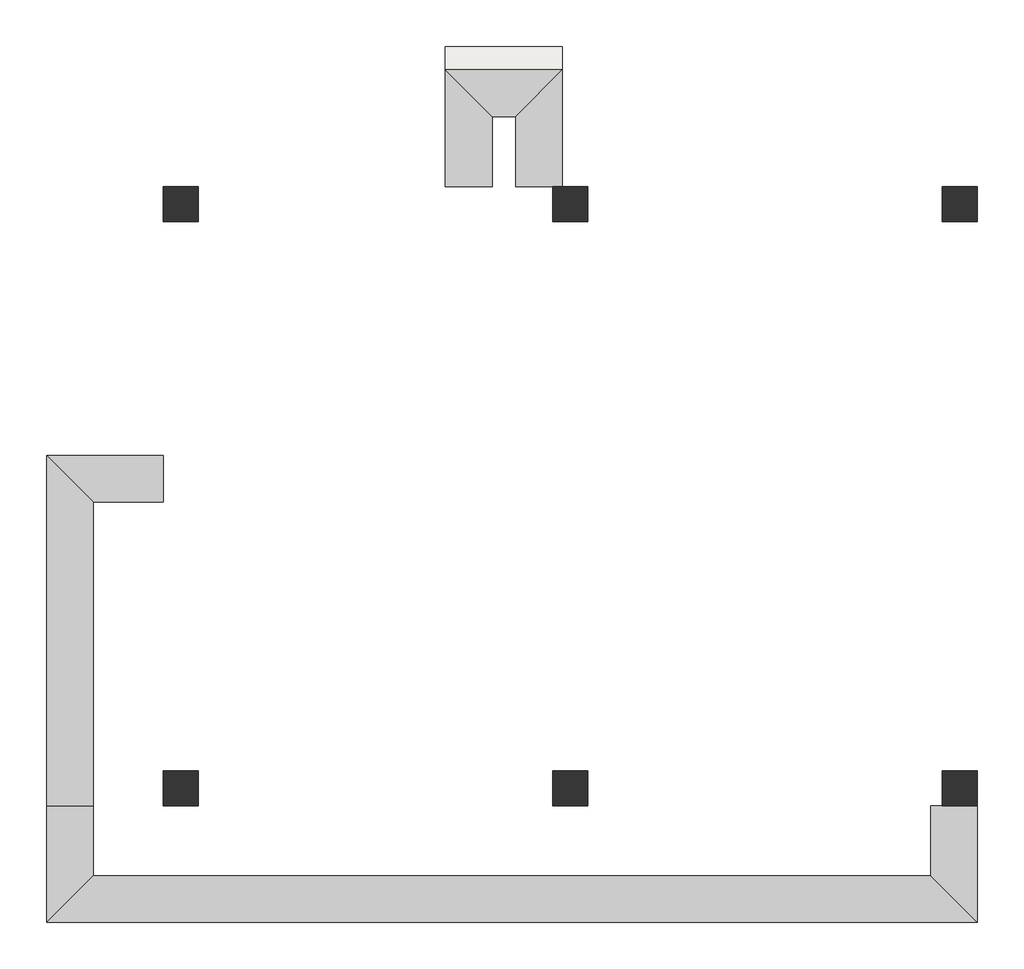
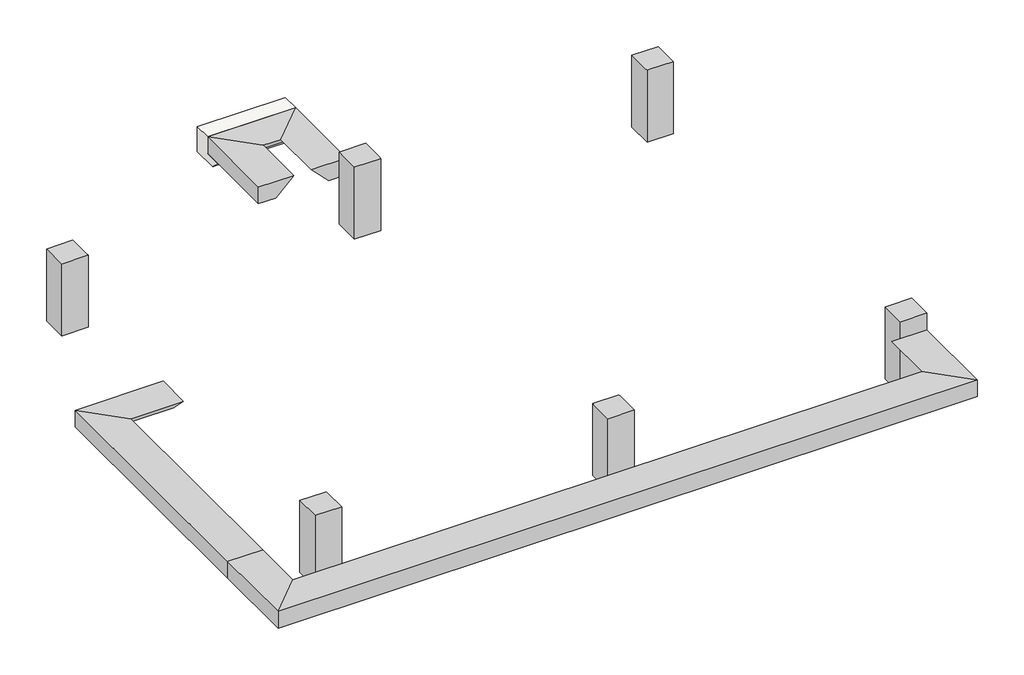
# One storey: 6 columns, 2 proxies, 1 slab.
"""IFC4 building model written with IfcOpenShell, lengths in millimetres."""

import ifcopenshell
import ifcopenshell.guid

model = None  # the IFC model being written
_history = None  # IfcOwnerHistory: only IFC2X3 demands one
_inside = {}  # id of a spatial element -> (the spatial element, [elements in it])
_under = {}  # id of a project, library or spatial element -> (it, [spatial elements below it])
_declared = {}  # id of a project -> (the project, [libraries it declares])
_typed = {}  # id of a type object -> (the type object, [elements of that type])
_made_of = {}  # id of a material, layer set ... -> (it, [elements and type objects made of it])


def new_model(schema):
    """Start an empty IFC model of exactly this schema.

    Asked for "IFC4X3", IfcOpenShell would pick the latest addendum, in which some entities
    have other attributes; the version numbers below select the first issue.
    IFC2X3 requires an IfcOwnerHistory on every rooted entity: one is made here for all.
    """
    global model, _history
    if schema == "IFC4X3":
        model = ifcopenshell.file(schema_version=(4, 3, 0, 0))
    else:
        model = ifcopenshell.file(schema=schema)
    _inside.clear()
    _under.clear()
    _declared.clear()
    _typed.clear()
    _made_of.clear()
    _history = None
    if model.schema == "IFC2X3":
        org = make("IfcOrganization", Name="unknown")
        user = make(
            "IfcPersonAndOrganization",
            ThePerson=make("IfcPerson", FamilyName="unknown"),
            TheOrganization=org,
        )
        app = make(
            "IfcApplication",
            ApplicationDeveloper=org,
            Version="unknown",
            ApplicationFullName="unknown",
            ApplicationIdentifier="unknown",
        )
        _history = make(
            "IfcOwnerHistory",
            OwningUser=user,
            OwningApplication=app,
            ChangeAction="ADDED",
            CreationDate=0,
        )
    return model


def make(cls, **values):
    """One entity of the class cls with the attributes given. An attribute that is None is left unset."""
    return model.create_entity(
        cls, **{name: value for name, value in values.items() if value is not None}
    )


def rooted(cls, **values):
    """An entity with a GlobalId (a new one), such as an element, a storey or a relation."""
    return make(cls, GlobalId=ifcopenshell.guid.new(), OwnerHistory=_history, **values)


def si_unit(unit_type, name, prefix=None):
    """IfcSIUnit, for example si_unit("LENGTHUNIT", "METRE", prefix="MILLI")."""
    return make("IfcSIUnit", UnitType=unit_type, Prefix=prefix, Name=name)


def assignment(units):
    """IfcUnitAssignment: the units of a project."""
    return None if units is None else make("IfcUnitAssignment", Units=units)


def point(xyz):
    """IfcCartesianPoint."""
    return None if xyz is None else make("IfcCartesianPoint", Coordinates=xyz)


def direction(xyz):
    """IfcDirection."""
    return None if xyz is None else make("IfcDirection", DirectionRatios=xyz)


def frame(location, z_axis=None, x_axis=None):
    """IfcAxis2Placement3D, a coordinate frame: its origin and axes. An axis left out is left unset."""
    return make(
        "IfcAxis2Placement3D",
        Location=point(location),
        Axis=direction(z_axis),
        RefDirection=direction(x_axis),
    )


def origin():
    """The frame at (0, 0, 0) with its axes left unset."""
    return frame((0.0, 0.0, 0.0))


def place(relative_to, where):
    """IfcLocalPlacement: puts the frame where relative to a parent placement (None: the world)."""
    return make(
        "IfcLocalPlacement", PlacementRelTo=relative_to, RelativePlacement=where
    )


def context(
    kind, dimensions, precision=None, world=None, true_north=None, identifier=None
):
    """IfcGeometricRepresentationContext, for example the 3D "Model" context."""
    return make(
        "IfcGeometricRepresentationContext",
        ContextIdentifier=identifier,
        ContextType=kind,
        CoordinateSpaceDimension=dimensions,
        Precision=precision,
        WorldCoordinateSystem=world,
        TrueNorth=true_north,
    )


def project(units=None, contexts=None):
    """IfcProject with its units and contexts."""
    return rooted(
        "IfcProject",
        Name="project",
        RepresentationContexts=contexts,
        UnitsInContext=assignment(units),
    )


def spatial(cls, under=None, at=None, **own):
    """A site, building, storey or space (cls), placed at a placement, below another one or the project."""
    s = rooted(cls, ObjectPlacement=at, **own)
    if under is not None:
        _under.setdefault(under.id(), (under, []))[1].append(s)
    return s


def polyline(points):
    """IfcPolyline through the points."""
    return make("IfcPolyline", Points=[point(p) for p in points])


def outline(outer, holes=None, kind="AREA"):
    """IfcArbitraryClosedProfileDef: a profile drawn as a closed curve; with holes, ...WithVoids."""
    if holes is None:
        return make("IfcArbitraryClosedProfileDef", ProfileType=kind, OuterCurve=outer)
    return make(
        "IfcArbitraryProfileDefWithVoids",
        ProfileType=kind,
        OuterCurve=outer,
        InnerCurves=holes,
    )


def extrude(swept, where, along, depth):
    """IfcExtrudedAreaSolid: the profile swept, set in the frame where, extruded along a direction by depth."""
    return make(
        "IfcExtrudedAreaSolid",
        SweptArea=swept,
        Position=where,
        ExtrudedDirection=direction(along),
        Depth=depth,
    )


def faces_of(points, faces, orient=None, outer=None):
    """IfcFace entities. A face is a list of loops; a loop is a list of indices into points, from 0.

    orient and outer hold one flag for each loop. By default every Orientation is true, the
    first loop of a face is its IfcFaceOuterBound and the others are IfcFaceBound.
    """
    made = []
    for i, loops in enumerate(faces):
        bounds = []
        for j, loop in enumerate(loops):
            is_outer = j == 0 if outer is None else outer[i][j]
            bounds.append(
                make(
                    "IfcFaceOuterBound" if is_outer else "IfcFaceBound",
                    Bound=make("IfcPolyLoop", Polygon=[points[k] for k in loop]),
                    Orientation=True if orient is None else orient[i][j],
                )
            )
        made.append(make("IfcFace", Bounds=bounds))
    return made


def faceted_brep(points, faces, orient=None, outer=None, voids=None):
    """IfcFacetedBrep: a solid bounded by flat faces; with voids (closed shells), ...WithVoids."""
    shared = [point(p) for p in points]
    hull = make("IfcClosedShell", CfsFaces=faces_of(shared, faces, orient, outer))
    if voids is None:
        return make("IfcFacetedBrep", Outer=hull)
    return make(
        "IfcFacetedBrepWithVoids",
        Outer=hull,
        Voids=[
            make(cls, CfsFaces=faces_of(shared, fs, o, b)) for cls, fs, o, b in voids
        ],
    )


def shape(context_of_items, identifier, shape_type, items):
    """IfcShapeRepresentation: the items that make up one representation, for example the "Body"."""
    return make(
        "IfcShapeRepresentation",
        ContextOfItems=context_of_items,
        RepresentationIdentifier=identifier,
        RepresentationType=shape_type,
        Items=items,
    )


def made_of(thing, what):
    """Note that an element or type object is made of a material, layer set ...; save() writes the relation."""
    if what is not None:
        _made_of.setdefault(what.id(), (what, []))[1].append(thing)
    return thing


def element(
    cls,
    number,
    at=None,
    inside=None,
    cuts=None,
    type_object=None,
    material=None,
    context=None,
    identifier="Body",
    shape_type=None,
    held_by="IfcProductDefinitionShape",
    body=None,
    shapes=None,
    **own,
):
    """One element of the class cls, such as IfcWall. Its Tag is "e" and its number.

    at: its placement. inside: the storey or other place that contains it. cuts: it is an
    opening in that element (IfcRelVoidsElement). A single representation is given by context,
    identifier, shape_type and body (its items); several are given by shapes. held_by: the class
    of the entity that holds the representations. save() writes the other relations.
    """
    e = rooted(cls, Tag="e%d" % number, ObjectPlacement=at, **own)
    if body is not None:
        shapes = [shape(context, identifier, shape_type, body)]
    if shapes is not None:
        e.Representation = make(held_by, Representations=shapes)
    if inside is not None:
        _inside.setdefault(inside.id(), (inside, []))[1].append(e)
    if cuts is not None:
        rooted(
            "IfcRelVoidsElement", RelatingBuildingElement=cuts, RelatedOpeningElement=e
        )
    if type_object is not None:
        _typed.setdefault(type_object.id(), (type_object, []))[1].append(e)
    return made_of(e, material)


def aggregate(whole, parts):
    """IfcRelAggregates: a whole, such as a stair, and the parts it consists of."""
    return rooted("IfcRelAggregates", RelatingObject=whole, RelatedObjects=parts)


def save(model, path):
    """Write the relations noted so far, then the file.

    IfcRelAggregates (storeys below a building ...), IfcRelContainedInSpatialStructure (elements
    in a storey), IfcRelDefinesByType, IfcRelAssociatesMaterial and IfcRelDeclares: one each for
    every whole, place, type object, material and project.
    """
    for whole, parts in _under.values():
        aggregate(whole, parts)
    for where, things in _inside.values():
        rooted(
            "IfcRelContainedInSpatialStructure",
            RelatedElements=things,
            RelatingStructure=where,
        )
    for kind, things in _typed.values():
        rooted("IfcRelDefinesByType", RelatedObjects=things, RelatingType=kind)
    for what, things in _made_of.values():
        rooted("IfcRelAssociatesMaterial", RelatedObjects=things, RelatingMaterial=what)
    for by, libraries in _declared.values():
        rooted("IfcRelDeclares", RelatingContext=by, RelatedDefinitions=libraries)
    model.write(path)


model = new_model("IFC4")

# Units and contexts
model_context = context("Model", 3, world=origin())
ifc_project = project(units=[si_unit("LENGTHUNIT", "METRE", prefix="MILLI")], contexts=[model_context])

# Site, building, storey
site = spatial("IfcSite", under=ifc_project)
building = spatial("IfcBuilding", under=site)
storey = spatial("IfcBuildingStorey", under=building, Name="T.O.C_-1,300", Elevation=-1300.0)

# Proxies
placement = place(None, origin())
element("IfcBuildingElementProxy", 1, Name="Slab Edge", ObjectType="Slab Edge", at=placement, inside=storey, context=model_context, shape_type="Brep", body=[
    faceted_brep([(10225.0, 13274.5208589, -600.0), (9925.0, 13274.5208589, -600.0), (9625.0, 13274.5208589, -300.0), (10225.0, 13274.5208589, -300.0), (10225.0, 11774.5208589, -300.0), (10225.0, 11774.5208589, -600.0), (9625.0, 12374.5208589, -300.0), (9925.0, 12074.5208589, -600.0), (-1725.0, 11774.5208589, -300.0), (-1725.0, 11774.5208589, -600.0), (-1125.0, 12374.5208589, -300.0), (-1425.0, 12074.5208589, -600.0), (-1725.0, 17774.5208589, -300.0), (-1725.0, 17774.5208589, -600.0), (-1725.0, 13274.5208589, -600.0), (-1725.0, 13274.5208589, -300.0), (-1125.0, 17174.5208589, -300.0), (-1125.0, 13274.5208589, -300.0), (-1425.0, 17474.5208589, -600.0), (-1425.0, 13274.5208589, -600.0), (-225.0, 17774.5208589, -600.0), (-225.0, 17774.5208589, -300.0), (-225.0, 17174.5208589, -300.0), (-225.0, 17474.5208589, -600.0)], [[[0, 1, 2, 3]], [[4, 5, 0, 3]], [[6, 4, 3, 2]], [[7, 6, 2, 1]], [[5, 7, 1, 0]], [[8, 9, 5, 4]], [[10, 8, 4, 6]], [[11, 10, 6, 7]], [[9, 11, 7, 5]], [[12, 13, 14, 15]], [[16, 12, 15, 17]], [[18, 16, 17, 19]], [[13, 18, 19, 14]], [[15, 14, 9, 8]], [[17, 15, 8, 10]], [[19, 17, 10, 11]], [[14, 19, 11, 9]], [[20, 21, 22, 23]], [[21, 20, 13, 12]], [[22, 21, 12, 16]], [[23, 22, 16, 18]], [[20, 23, 18, 13]]]),
])
element("IfcBuildingElementProxy", 2, Name="Slab Edge", ObjectType="Slab Edge", at=placement, inside=storey, context=model_context, shape_type="Brep", body=[
    faceted_brep([(4895.0, 21224.5208589, -450.0), (4895.0, 21224.5208589, -150.0), (4295.0, 21224.5208589, -150.0), (4595.0, 21224.5208589, -450.0), (4895.0, 22724.5208589, -450.0), (4895.0, 22724.5208589, -150.0), (4295.0, 22124.5208589, -150.0), (4595.0, 22424.5208589, -450.0), (3395.0, 22724.5208589, -450.0), (3395.0, 22724.5208589, -150.0), (3995.0, 22124.5208589, -150.0), (3695.0, 22424.5208589, -450.0), (3395.0, 21224.5208589, -450.0), (3695.0, 21224.5208589, -450.0), (3995.0, 21224.5208589, -150.0), (3395.0, 21224.5208589, -150.0)], [[[0, 1, 2, 3]], [[1, 0, 4, 5]], [[2, 1, 5, 6]], [[3, 2, 6, 7]], [[0, 3, 7, 4]], [[5, 4, 8, 9]], [[6, 5, 9, 10]], [[7, 6, 10, 11]], [[4, 7, 11, 8]], [[12, 13, 14, 15]], [[9, 8, 12, 15]], [[10, 9, 15, 14]], [[11, 10, 14, 13]], [[8, 11, 13, 12]]]),
])

# Columns
element("IfcColumn", 3, ObjectType="Concrete-Rectangular-Column : CL111_450x450", at=placement, inside=storey, context=model_context, shape_type="Brep", body=[
    faceted_brep([(225.0, 13724.5208589, -1300.0), (225.0, 13274.5208589, -1300.0), (-225.0, 13274.5208589, -1300.0), (-225.0, 13724.5208589, -1300.0), (225.0, 13724.5208589, 0.0), (225.0, 13674.5208589, 0.0), (225.0, 13274.5208589, 0.0), (225.0, 13274.5208589, -600.0), (-225.0, 13274.5208589, 0.0), (-225.0, 13724.5208589, 0.0), (-225.0, 13724.5208589, -600.0), (175.0, 13724.5208589, 0.0)], [[[0, 1, 2, 3]], [[4, 5, 6, 7, 1, 0]], [[6, 8, 2, 1, 7]], [[8, 9, 10, 3, 2]], [[9, 11, 4, 0, 3, 10]], [[4, 11, 9, 8, 6, 5]]]),
])
element("IfcColumn", 4, ObjectType="Concrete-Rectangular-Column : CL111_450x450", at=placement, inside=storey, context=model_context, shape_type="Brep", body=[
    faceted_brep([(5225.0, 13724.5208589, -1300.0), (5225.0, 13274.5208589, -1300.0), (4775.0, 13274.5208589, -1300.0), (4775.0, 13724.5208589, -1300.0), (5225.0, 13724.5208589, 0.0), (5225.0, 13674.5208589, 0.0), (5225.0, 13274.5208589, 0.0), (5225.0, 13274.5208589, -600.0), (4775.0, 13274.5208589, 0.0), (4775.0, 13274.5208589, -600.0), (4775.0, 13674.5208589, 0.0), (4775.0, 13724.5208589, 0.0)], [[[0, 1, 2, 3]], [[4, 5, 6, 7, 1, 0]], [[6, 8, 9, 2, 1, 7]], [[8, 10, 11, 3, 2, 9]], [[11, 4, 0, 3]], [[4, 11, 10, 8, 6, 5]]]),
])
element("IfcColumn", 5, ObjectType="Concrete-Rectangular-Column : CL111_450x450", at=placement, inside=storey, context=model_context, shape_type="Brep", body=[
    faceted_brep([(10225.0, 13724.5208589, -1300.0), (10225.0, 13274.5208589, -1300.0), (9775.0, 13274.5208589, -1300.0), (9775.0, 13724.5208589, -1300.0), (10225.0, 13724.5208589, 0.0), (10225.0, 13274.5208589, 0.0), (10225.0, 13724.5208589, -600.0), (9775.0, 13274.5208589, 0.0), (9775.0, 13274.5208589, -600.0), (9775.0, 13674.5208589, 0.0), (9775.0, 13724.5208589, 0.0), (9825.0, 13724.5208589, 0.0)], [[[0, 1, 2, 3]], [[4, 5, 1, 0, 6]], [[5, 7, 8, 2, 1]], [[7, 9, 10, 3, 2, 8]], [[10, 11, 4, 6, 0, 3]], [[4, 11, 10, 9, 7, 5]]]),
])
element("IfcColumn", 6, ObjectType="Concrete-Rectangular-Column : CL111_450x450", at=placement, inside=storey, context=model_context, shape_type="Brep", body=[
    faceted_brep([(10225.0, 21224.5208589, -1300.0), (10225.0, 20774.5208589, -1300.0), (9775.0, 20774.5208589, -1300.0), (9775.0, 21224.5208589, -1300.0), (10225.0, 21224.5208589, 0.0), (10225.0, 20774.5208589, 0.0), (10225.0, 20774.5208589, -600.0), (9825.0, 20774.5208589, 0.0), (9775.0, 20774.5208589, 0.0), (9775.0, 20824.5208589, 0.0), (9775.0, 21224.5208589, 0.0), (9775.0, 21224.5208589, -600.0)], [[[0, 1, 2, 3]], [[4, 5, 6, 1, 0]], [[5, 7, 8, 2, 1, 6]], [[8, 9, 10, 11, 3, 2]], [[10, 4, 0, 3, 11]], [[4, 10, 9, 8, 7, 5]]]),
])
element("IfcColumn", 7, ObjectType="Concrete-Rectangular-Column : CL111_450x450", at=placement, inside=storey, context=model_context, shape_type="Brep", body=[
    faceted_brep([(5225.0, 21224.5208589, -1300.0), (5225.0, 20774.5208589, -1300.0), (4775.0, 20774.5208589, -1300.0), (4775.0, 21224.5208589, -1300.0), (5225.0, 21224.5208589, 0.0), (5225.0, 20824.5208589, 0.0), (5225.0, 20774.5208589, 0.0), (5225.0, 21224.5208589, -600.0), (4775.0, 20774.5208589, 0.0), (4775.0, 21224.5208589, 0.0)], [[[0, 1, 2, 3]], [[4, 5, 6, 1, 0, 7]], [[6, 8, 2, 1]], [[8, 9, 3, 2]], [[9, 4, 7, 0, 3]], [[4, 9, 8, 6, 5]]]),
])
element("IfcColumn", 8, ObjectType="Concrete-Rectangular-Column : CL111_450x450", at=placement, inside=storey, context=model_context, shape_type="Brep", body=[
    faceted_brep([(225.0, 21224.5208589, -1300.0), (225.0, 20774.5208589, -1300.0), (-225.0, 20774.5208589, -1300.0), (-225.0, 21224.5208589, -1300.0), (225.0, 21224.5208589, 0.0), (225.0, 20824.5208589, 0.0), (225.0, 20774.5208589, 0.0), (225.0, 21224.5208589, -600.0), (175.0, 20774.5208589, 0.0), (-225.0, 20774.5208589, 0.0), (-225.0, 20774.5208589, -600.0), (-225.0, 21224.5208589, 0.0)], [[[0, 1, 2, 3]], [[4, 5, 6, 1, 0, 7]], [[6, 8, 9, 10, 2, 1]], [[9, 11, 3, 2, 10]], [[11, 4, 7, 0, 3]], [[4, 11, 9, 8, 6, 5]]]),
])

# Slab
element("IfcSlab", 9, ObjectType="STOOP_SLAB EDGE(계단부분) : STOOP_SLAB EDGE(계단부분)", at=placement, inside=storey, context=model_context, shape_type="SweptSolid", body=[
    extrude(outline(polyline([(23024.5208589, -150.0), (23024.5208589, -600.0), (22574.5208589, -600.0), (22424.5208589, -450.0), (22724.5208589, -450.0), (22724.5208589, -150.0), (23024.5208589, -150.0)])), frame((3393.3757722, 0.0, 0.0), z_axis=(1.0, 0.0, 0.0), x_axis=(0.0, 1.0, 0.0)), (0.0, 0.0, 1.0), 1501.6242278),
])

save(model, "model.ifc")

# Revit data of these elements
# Project information
#   Building Name = "Main Gate Security"
#   Project Status = "Project Status"
#   Client Name = "현대엔지니어링"
#   Project Address = "서울시 종로구 율곡로 75(계동)"
#   Project Name = "Therma Visayas Energy Project"
#   Project Number = "001"
# Grids (mm)
#   "B": line (5000, 25626.165) -> (5000, 10142.075)
#   "C": line (10000, 25626.165) -> (10000, 10142.075)
#   "A": line (0, 25626.165) -> (0, 10142.075)
#   "5": line (3500, 10142.075) -> (3500, 25626.165)
#   "6": line (7500, 10142.075) -> (7500, 25626.165)
#   "10": line (14956.387, 18199.521) -> (-5363.617, 18199.521)
#   "1": line (-5363.617, 13499.521) -> (13263.593, 13499.521)
#   "2": line (-5363.617, 20999.521) -> (13263.593, 20999.521)
# Type "Concrete-Rectangular-Column : CL111_450x450"
#   Description = "UG 철골 기둥용 Pedestal"
#   b = 450 mm
#   h = 450 mm
#   hec_material3 [instance default] = none
#   hec_material2 [instance default] = A03AE056-00001_Bitumen/Bituminous/Asphalt Coating
#   hec_material1 [instance default] = A03AC035-00001_Form Work (3 times in use)_Flat
#   Structural Material [instance default] = A03AC032-00007_Structural Concrete_Type1_25MPa-30Mpa
# Type "STOOP_SLAB EDGE(계단부분) : STOOP_SLAB EDGE(계단부분)"
#   built-in parameter 1001306 [instance default] = 3.93701 (stored number, unit not read)
#   Default Elevation = 0
#   Structural Material = none
# Elements 1, 2 (IfcBuildingElementProxy, "Slab Edge")
#   W11) Activity ID = "C02AGB040"
#   W12) Activity Name = "Main Gate Security Building ‐ Exterior & Finish Work"
#   W13) Plan Start Date = "2017-01-12"
#   W14) Plan Finish Date = "2017-04-11"
#   W15) Duration = "71"
#   W16) Actual Start Date = "2017-01-12"
#   W17) Actual Finish Date = "2017-04-11"
#   Phase Created = New Construction
#   Materials on its faces: "A03AD032-00007_Structural Concrete_25MPa-30MPa"
# Elements 3, 4, 5, 6, 7 (IfcColumn, "Concrete-Rectangular-Column : CL111_450x450")
#   Comments = ""
#   F01) Building Name = "Main Gate House"
#   F11) Project Building Tag_Type-1 = "Common"
#   F12) Project Building Tag_Type-2 = "Common"
#   F13) Project Facility Code = "Facility Code"
#   F21) Structural Type = "Concrete"
#   F31) Standard Building Code = "IBC"
#   F41) Discipline = "AR"
#   F51) Plan Start Date-Engineering = "2015-01-01"
#   F52) Plan Finish Date-Engineering = "2015-12-31"
#   F53) Duration = "365"
#   F54) Actual Start Date-Engineering = "2015-01-01"
#   F55) Actual Finish Date-Engineering = "2015-12-31"
#   F61) Plan Start Date-Construction = "2016-08-19"
#   F62) Plan Finish Date-Construction = "2017-01-31"
#   F64) Actual Start Date-Construction = "2016-08-19"
#   F63) Duration = "202"
#   F65) Actual Finish Date-Construction = "2017-01-31"
#   F91) Plant Type = "CFPP"
#   F92) KKS Structures, Building = "UYF"
#   P01) Project Name = "TVEP"
#   P02) Project Configuration = "CFB Boiler x 2(Foster Wheeler) + STG x 2(Alstom, 150MW)"
#   P03) Project Abbreviation = "TVEP"
#   P04) Project Code = "BEPH1402"
#   P05) Project Stage = "In operation"
#   P06) Project Location = "Sito Looc, Barangay Bato, Toledo City in Philippines"
#   P07) Project Owner = "Therma Visayas, Inc."
#   P08) Project O.E = "Flour"
#   P09) Project Schedule = "ITB Issueing Date : 2013.07.30\r\nSite Survey : 2013.08.19-20\r\nBid Closing Date : 2013.11.29\r\nPreferred Bidder Notice 접수 : 2014.04.27\r\nTarget award date : 2014 05\r\nLOA 접수 : 2014.05.21\r\nSigning Ceremony : 2014.05.30"
#   P10) Basic Wind Speed = "55.6 m/s"
#   P11) Seismic = "NSCP 2010, Zone 4 (PGA : 0.4g)"
#   P12) Soil = "Sc"
#   P13) Soil Capacity = "100kN/m2"
#   P14) Pile Capacity = "PHC(D400) : 1200kN"
#   W00) Work Master Code = "A03AC032-00007"
#   W01) Work Master_Lv1 = "Concrete Work"
#   W02) Work Master_Lv2 = "Substructure Work"
#   W03) Work Master_Spec.1 = "Structural Concrete"
#   W04) Work Master_Spec.2 = "Cement Type-1"
#   W05) Work Master_Spec.3 = "25MPa < F'c (Cylinder Strength) ≤ 30MPa"
#   W11) Activity ID = "C02AGB010"
#   W12) Activity Name = "Main Gate Security Building ‐ Building Foundaton"
#   W13) Plan Start Date = "2016-08-19"
#   W14) Plan Finish Date = "2016-09-22"
#   W15) Duration = "26"
#   W16) Actual Start Date = "2016-08-19"
#   W17) Actual Finish Date = "2016-09-22"
#   R02) Unit Price = 0
#   Structural Material = A03AD032-00007_Structural Concrete_25MPa-30MPa
#   hec_material3 = none
#   hec_material2 = none
#   hec_material1 = none
#   Phase Created = New Construction
#   Materials on its faces: "A03AD032-00007_Structural Concrete_25MPa-30MPa"
# Element 8 (IfcColumn, "Concrete-Rectangular-Column : CL111_450x450")
#   Comments = ""
#   F01) Building Name = "Main Gate House"
#   F11) Project Building Tag_Type-1 = "Common"
#   F12) Project Building Tag_Type-2 = "Common"
#   F13) Project Facility Code = "Facility Code"
#   F21) Structural Type = "Concrete"
#   F31) Standard Building Code = "IBC"
#   F41) Discipline = "AR"
#   F51) Plan Start Date-Engineering = "2015-01-01"
#   F52) Plan Finish Date-Engineering = "2015-12-31"
#   F53) Duration = "365"
#   F54) Actual Start Date-Engineering = "2015-01-01"
#   F55) Actual Finish Date-Engineering = "2015-12-31"
#   F61) Plan Start Date-Construction = "2016-08-19"
#   F62) Plan Finish Date-Construction = "2017-01-31"
#   F64) Actual Start Date-Construction = "2016-08-19"
#   F63) Duration = "202"
#   F65) Actual Finish Date-Construction = "2017-01-31"
#   F91) Plant Type = "CFPP"
#   F92) KKS Structures, Building = "UYF"
#   P01) Project Name = "TVEP"
#   P02) Project Configuration = "CFB Boiler x 2(Foster Wheeler) + STG x 2(Alstom, 150MW)"
#   P03) Project Abbreviation = "TVEP"
#   P04) Project Code = "BEPH1402"
#   P05) Project Stage = "In operation"
#   P06) Project Location = "Sito Looc, Barangay Bato, Toledo City in Philippines"
#   P07) Project Owner = "Therma Visayas, Inc."
#   P08) Project O.E = "Flour"
#   P09) Project Schedule = "ITB Issueing Date : 2013.07.30\r\nSite Survey : 2013.08.19-20\r\nBid Closing Date : 2013.11.29\r\nPreferred Bidder Notice 접수 : 2014.04.27\r\nTarget award date : 2014 05\r\nLOA 접수 : 2014.05.21\r\nSigning Ceremony : 2014.05.30"
#   P10) Basic Wind Speed = "55.6 m/s"
#   P11) Seismic = "NSCP 2010, Zone 4 (PGA : 0.4g)"
#   P12) Soil = "Sc"
#   P13) Soil Capacity = "100kN/m2"
#   P14) Pile Capacity = "PHC(D400) : 1200kN"
#   W00) Work Master Code = "A03AC032-00007"
#   W01) Work Master_Lv1 = "Concrete Work"
#   W02) Work Master_Lv2 = "Substructure Work"
#   W03) Work Master_Spec.1 = "Structural Concrete"
#   W04) Work Master_Spec.2 = "Cement Type-1"
#   W05) Work Master_Spec.3 = "25MPa < F'c (Cylinder Strength) ≤ 30MPa"
#   W11) Activity ID = "C02AGB010"
#   W12) Activity Name = "Main Gate Security Building ‐ Building Foundaton"
#   W13) Plan Start Date = "2016-08-19"
#   W14) Plan Finish Date = "2016-09-22"
#   W15) Duration = "26"
#   W16) Actual Start Date = "2016-08-19"
#   W17) Actual Finish Date = "2016-09-22"
#   TMP_Element Name = "C1"
#   R02) Unit Price = 0
#   Structural Material = A03AD032-00007_Structural Concrete_25MPa-30MPa
#   hec_material3 = none
#   hec_material2 = none
#   hec_material1 = none
#   Phase Created = New Construction
#   Materials on its faces: "A03AD032-00007_Structural Concrete_25MPa-30MPa"
# Element 9 (IfcSlab, "STOOP_SLAB EDGE(계단부분) : STOOP_SLAB EDGE(계단부분)")
#   F01) Building Name = "Main Gate House"
#   F11) Project Building Tag_Type-1 = "Common"
#   F12) Project Building Tag_Type-2 = "Common"
#   F13) Project Facility Code = "Facility Code"
#   F21) Structural Type = "Concrete"
#   F31) Standard Building Code = "IBC"
#   F41) Discipline = "AR"
#   F51) Plan Start Date-Engineering = "2015-01-01"
#   F52) Plan Finish Date-Engineering = "2015-12-31"
#   F53) Duration = "365"
#   F54) Actual Start Date-Engineering = "2015-01-01"
#   F55) Actual Finish Date-Engineering = "2015-12-31"
#   F61) Plan Start Date-Construction = "2016-08-19"
#   F62) Plan Finish Date-Construction = "2017-01-31"
#   F64) Actual Start Date-Construction = "2016-08-19"
#   F63) Duration = "202"
#   F65) Actual Finish Date-Construction = "2017-01-31"
#   F91) Plant Type = "CFPP"
#   F92) KKS Structures, Building = "UYF"
#   P01) Project Name = "TVEP"
#   P02) Project Configuration = "CFB Boiler x 2(Foster Wheeler) + STG x 2(Alstom, 150MW)"
#   P03) Project Abbreviation = "TVEP"
#   P04) Project Code = "BEPH1402"
#   P05) Project Stage = "In operation"
#   P06) Project Location = "Sito Looc, Barangay Bato, Toledo City in Philippines"
#   P07) Project Owner = "Therma Visayas, Inc."
#   P08) Project O.E = "Flour"
#   P09) Project Schedule = "ITB Issueing Date : 2013.07.30\r\nSite Survey : 2013.08.19-20\r\nBid Closing Date : 2013.11.29\r\nPreferred Bidder Notice 접수 : 2014.04.27\r\nTarget award date : 2014 05\r\nLOA 접수 : 2014.05.21\r\nSigning Ceremony : 2014.05.30"
#   P10) Basic Wind Speed = "55.6 m/s"
#   P11) Seismic = "NSCP 2010, Zone 4 (PGA : 0.4g)"
#   P12) Soil = "Sc"
#   P13) Soil Capacity = "100kN/m2"
#   P14) Pile Capacity = "PHC(D400) : 1200kN"
#   W11) Activity ID = "C02AGB040"
#   W12) Activity Name = "Main Gate Security Building ‐ Exterior & Finish Work"
#   W13) Plan Start Date = "2017-01-12"
#   W14) Plan Finish Date = "2017-04-11"
#   W15) Duration = "71"
#   W16) Actual Start Date = "2017-01-12"
#   W17) Actual Finish Date = "2017-04-11"
#   R02) Unit Price = 0
#   built-in parameter 1001306 = 4.92659 (stored number, unit not read)
#   Phase Created = New Construction
# Materials
#   "A03AE056-00001_Bitumen/Bituminous/Asphalt Coating": class "Generic", colour RGB 17 17 17, transparency 0, Description = "Damp-proofing", W00) Work Master Code = "A03AE056-00001", W01) Work Master_Lv1 = "Concrete Work", W02) Work Master_Lv2 = "Concrete Protective Coating (U/G)", W03) Work Master_Spec.1 = "Bitumen/Bituminous/Asphalt Coating", Cost = 0
#   "A03AC035-00001_Form Work (3 times in use)_Flat": class "Wood", colour RGB 149 120 74, transparency 0, Description = "Plywood", W00) Work Master Code = "A03AC035-00001", W01) Work Master_Lv1 = "Concrete Work", W02) Work Master_Lv2 = "Substructure Work", W03) Work Master_Spec.1 = "Form Work (3 times in use)", W04) Work Master_Spec.2 = "Flat Form", W05) Work Master_Spec.3 = "Dressed Lumber, Plywood or Steel Form(Wood Planks are not Allowed) incl. Chamfer", Cost = 0
#   "A03AC032-00007_Structural Concrete_Type1_25MPa-30Mpa": class "Concrete", colour RGB 176 176 176, transparency 0, Keynote = "09910.A1", Description = "Reinf. Conc.", W00) Work Master Code = "A03AC032-00007", W01) Work Master_Lv1 = "Concrete Work", W02) Work Master_Lv2 = "Substructure Work", W03) Work Master_Spec.1 = "Structural Concrete", W04) Work Master_Spec.2 = "Cement Type-1", W05) Work Master_Spec.3 = "25MPa < F'c (Cylinder Strength) ≤ 30MPa", Cost = 0
#   "A03AD032-00007_Structural Concrete_25MPa-30MPa": class "Concrete", colour RGB 176 176 176, transparency 0, Keynote = "09910.A1", Description = "Reinf. Conc.", W00) Work Master Code = "A03AD032-00007", W01) Work Master_Lv1 = "Concrete Work", W02) Work Master_Lv2 = "Superstructure Work", W03) Work Master_Spec.1 = "Structural Concrete", W04) Work Master_Spec.2 = "Cement Type-1", W05) Work Master_Spec.3 = "25MPa < F'c (Cylinder Strength) ≤ 30MPa", Cost = 0
# Room, not placed, phase "New Construction", upper offset 0 mm, lower offset 0 mm
#   Comments = ""
#   Base Finish = "EXPOXY PAINT ON THK.15 CEMENT PLASTER(H=100)"
#   Ceiling Finish = "LATEX PAINT ON FAIR FACED CONC."
#   Wall Finish = "LATEX PAINT ON THK.15 CEMENT PLASTER + MASONRY WALL"
#   Floor Finish = "EPOXY PAINT ON STEEL TROWELED CONC. SLAB"
#   Number = "1"
#   Name = ""
#   F01) Building Name = "CENTRAL CONTROL BUILDING"
#   S01) Room Name = "CABLE ROOM"
#   S02) Room Number(Project) = "UCA01R0001"
# Room, not placed, phase "New Construction", upper offset 0 mm, lower offset 0 mm
#   Comments = ""
#   Number = "2"
#   Name = ""
#   S01) Room Name = ""
#   S02) Room Number(Project) = ""
